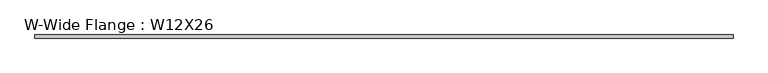
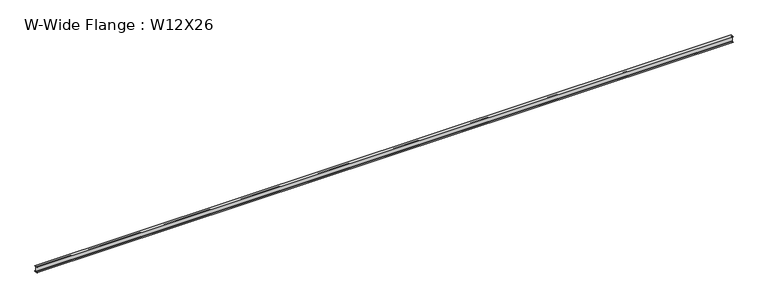
"""IFC4 building model written with IfcOpenShell, lengths in millimetres: beam geometry, W-Wide Flange : W12X26."""

from ifc_helpers import new_model, si_unit, point, frame, frame_2d, origin, place, context, project, spatial, polyline, circle_curve, trimmed, segment, composite_curve, outline, extrude, source, transform, mapped, element, save


def w_wide_flange_w12x26_89544ef1(model_context):
    return source(origin(), model_context, "Body", "SweptSolid", [
        extrude(outline(composite_curve([segment(polyline([(82.4011719, -145.5539063), (82.4011719, -155.178125), (-82.4011719, -155.178125), (-82.4011719, -145.5539063), (-20.2902344, -145.5539063)]), True, "CONTINUOUS"), segment(trimmed(circle_curve(frame_2d((-20.2902344, -128.190625)), 17.3632812), [point((-20.2902344, -145.5539063))], [point((-2.9269531, -128.190625))], True, "CARTESIAN"), True, "CONTINUOUS"), segment(polyline([(-2.9269531, -128.190625), (-2.9269531, 128.190625)]), True, "CONTINUOUS"), segment(trimmed(circle_curve(frame_2d((-20.2902344, 128.190625)), 17.3632812), [point((-2.9269531, 128.190625))], [point((-20.2902344, 145.5539062))], True, "CARTESIAN"), True, "CONTINUOUS"), segment(polyline([(-20.2902344, 145.5539062), (-82.4011719, 145.5539062), (-82.4011719, 155.178125), (82.4011719, 155.178125), (82.4011719, 145.5539062), (20.2902344, 145.5539062)]), True, "CONTINUOUS"), segment(trimmed(circle_curve(frame_2d((20.2902344, 128.190625)), 17.3632812), [point((20.2902344, 145.5539062))], [point((2.9269531, 128.190625))], True, "CARTESIAN"), True, "CONTINUOUS"), segment(polyline([(2.9269531, 128.190625), (2.9269531, -128.190625)]), True, "CONTINUOUS"), segment(trimmed(circle_curve(frame_2d((20.2902344, -128.190625)), 17.3632812), [point((2.9269531, -128.190625))], [point((20.2902344, -145.5539063))], True, "CARTESIAN"), True, "CONTINUOUS"), segment(polyline([(20.2902344, -145.5539063), (82.4011719, -145.5539063)]), True, "CONTINUOUS")], self_intersect=False)), frame((-18440.6993086, 0.0, 0.0), z_axis=(1.0, 0.0, 0.0), x_axis=(0.0, 1.0, 0.0)), (0.0, 0.0, 1.0), 36978.2361173),
    ])


if __name__ == "__main__":
    model = new_model("IFC4")
    model_context = context("Model", 3, world=origin())
    ifc_project = project(units=[si_unit("LENGTHUNIT", "METRE", prefix="MILLI")], contexts=[model_context])
    site = spatial("IfcSite", under=ifc_project)
    building = spatial("IfcBuilding", under=site)
    placement = place(None, origin())
    w_wide_flange_w12x26_shape = w_wide_flange_w12x26_89544ef1(model_context)
    element("IfcBeam", 1, ObjectType="W-Wide Flange : W12X26", at=placement, inside=building, context=model_context, shape_type="MappedRepresentation", body=[
        mapped(w_wide_flange_w12x26_shape, transform((0.0, 0.0, 0.0), x_axis=(1.0, 0.0, 0.0), y_axis=(0.0, 1.0, 0.0), z_axis=(0.0, 0.0, 1.0))),
    ])
    save(model, "model.ifc")

# Revit data of these elements
# Type "W-Wide Flange : W12X26"
#   Assembly Code = "B10"
#   W = 26
#   Length [instance default] = 5' - 0"
#   bf = 0' - 6 125/256"
#   d = 1' - 0 7/32"
#   k = 0' - 1 1/16"
#   k2 = 0' - 0 175/256"
#   tf = 0' - 0 97/256"
#   tw = 0' - 0 59/256"
#   A = 0.053125 SF
#   Structural Material [instance default] = none
